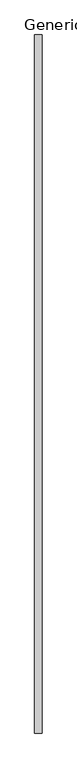
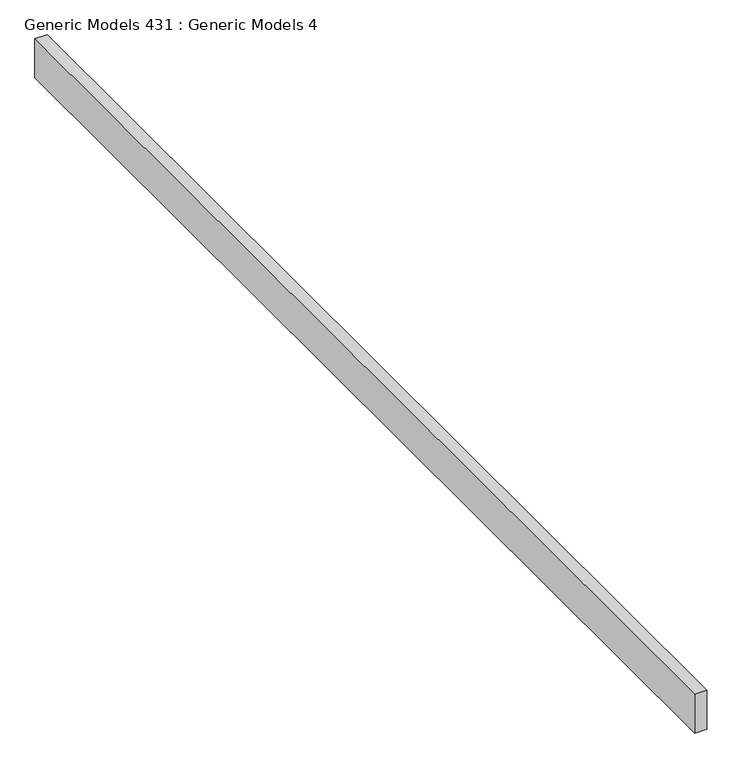
"""IFC4 building model written with IfcOpenShell, lengths in millimetres: proxy geometry, Generic Models 431 : Generic Models 4."""

from ifc_helpers import new_model, si_unit, frame, origin, place, context, project, spatial, polyline, outline, extrude, source, transform, mapped, element, save


def generic_models_431_generic_models_4_fb59ed78(model_context):
    return source(origin(), model_context, "Body", "SweptSolid", [
        extrude(outline(polyline([(8553.2763705, -6864.9230338), (8505.3973705, -6864.9230338), (8505.3973705, -2343.7230338), (8553.2763704, -2343.7230338), (8553.2763705, -6864.9230338)])), frame((0.0, 0.0, 126383.796), z_axis=(0.0, 0.0, 1.0), x_axis=(1.0, 0.0, 0.0)), (0.0, 0.0, 1.0), 162.0790924),
    ])


if __name__ == "__main__":
    model = new_model("IFC4")
    model_context = context("Model", 3, world=origin())
    ifc_project = project(units=[si_unit("LENGTHUNIT", "METRE", prefix="MILLI")], contexts=[model_context])
    site = spatial("IfcSite", under=ifc_project)
    building = spatial("IfcBuilding", under=site)
    placement = place(None, origin())
    generic_models_431_generic_models_4_shape = generic_models_431_generic_models_4_fb59ed78(model_context)
    element("IfcBuildingElementProxy", 1, Name="Generic Models 431 : Generic Models 4", ObjectType="Generic Models 431 : Generic Models 4", at=placement, inside=building, context=model_context, shape_type="MappedRepresentation", body=[
        mapped(generic_models_431_generic_models_4_shape, transform((0.0, 0.0, 0.0), x_axis=(1.0, 0.0, 0.0), y_axis=(0.0, 1.0, 0.0), z_axis=(0.0, 0.0, 1.0))),
    ])
    save(model, "model.ifc")

# Revit data of these elements
# Element 1 (IfcBuildingElementProxy, "Generic Models 431 : Generic Models 4")
#   Materials on its faces: "_2X BLOCKING AS REQUIRED"
# Materials
#   "_2X BLOCKING AS REQUIRED": class "Generic", colour RGB 177 130 114, transparency 0, Cost = 0
